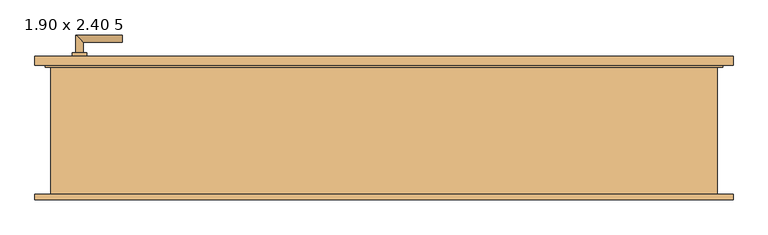
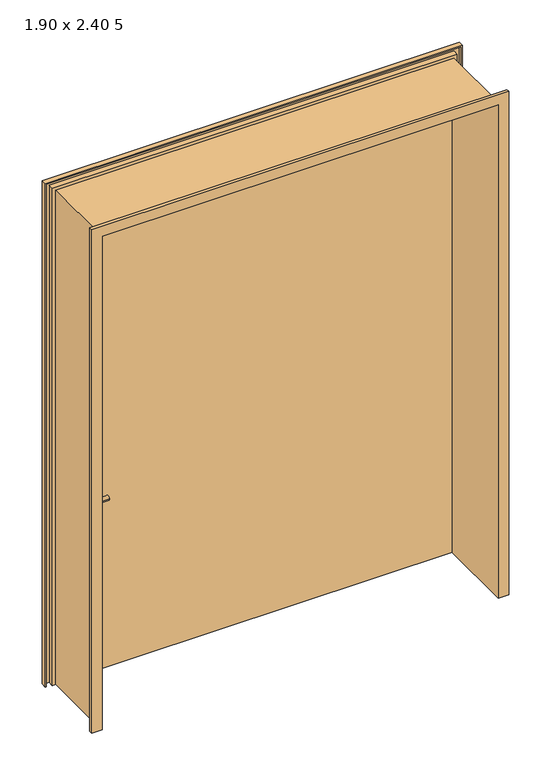
"""IFC4 building model written with IfcOpenShell, lengths in millimetres: door geometry, Drehflügel 1-flg - Stahlzarge : 1.90 x 2.40 5."""

from ifc_helpers import new_model, si_unit, point, frame, frame_2d, origin, place, context, project, spatial, polyline, circle_curve, ellipse_curve, trimmed, segment, composite_curve, outline, extrude, faceted_brep, source, transform, mapped, element, save
from ifc_brep_helpers import plane_surface, cylinder_surface, advanced_brep


def door_1_90_x_2_40_5_014a3839(model_context):
    return source(origin(), model_context, "Body", "SolidModel", [
        advanced_brep(
        [(-860.0, 169.4346141, 915.0), (-840.0, 169.4346141, 915.0), (-860.0, 99.4346141, 915.0), (-840.0, 119.4346141, 915.0), (-730.0, 99.4346141, 915.0), (-730.0, 119.4346141, 915.0)],
        [
            (0, 1, circle_curve(frame((-850.0, 169.4346141, 915.0), z_axis=(0.0, 1.0, 0.0), x_axis=(1.0, 0.0, 0.0)), 10.0)),
            (1, 0, circle_curve(frame((-850.0, 169.4346141, 915.0), z_axis=(0.0, 1.0, 0.0), x_axis=(1.0, 0.0, 0.0)), 10.0)),
            (0, 2),
            (2, 3, ellipse_curve(frame((-850.0, 109.4346141, 915.0), z_axis=(-0.7071067811865385, 0.7071067811865565, 0.0), x_axis=(0.7071067811865563, 0.7071067811865386, 0.0)), 14.1421356, 10.0)),
            (3, 1),
            (3, 2, ellipse_curve(frame((-850.0, 109.4346141, 915.0), z_axis=(-0.7071067811865385, 0.7071067811865565, 0.0), x_axis=(0.7071067811865563, 0.7071067811865386, 0.0)), 14.1421356, 10.0)),
            (4, 5, circle_curve(frame((-730.0, 109.4346141, 915.0), z_axis=(1.0, 0.0, 0.0), x_axis=(0.0, 1.0, 0.0)), 10.0)),
            (5, 4, circle_curve(frame((-730.0, 109.4346141, 915.0), z_axis=(1.0, 0.0, 0.0), x_axis=(0.0, 1.0, 0.0)), 10.0)),
            (2, 4),
            (5, 3),
        ],
        [
            plane_surface(frame((-850.0, 169.4346141, -372.7526403), z_axis=(0.0, 1.0, 0.0), x_axis=(0.0, 0.0, 1.0))),
            cylinder_surface(frame((-850.0, 169.4346141, 915.0), z_axis=(0.0, 1.0, 0.0), x_axis=(1.0, 0.0, 0.0)), 10.0),
            plane_surface(frame((-730.0, 109.4346141, -372.7526403), z_axis=(1.0, 0.0, 0.0), x_axis=(0.0, 0.0, 1.0))),
            cylinder_surface(frame((-850.0, 109.4346141, 915.0), z_axis=(-1.0, 0.0, 0.0), x_axis=(0.0, 1.0, 0.0)), 10.0),
        ],
        [
            (0, [[1, 2]]),
            (1, [[-1, 3, 4, 5]]),
            (1, [[-2, -5, 6, -3]]),
            (2, [[7, 8]]),
            (3, [[-4, 9, -8, 10]]),
            (3, [[-6, -10, -7, -9]]),
        ],
    ),
        advanced_brep(
        [(-840.0, 229.4346141, 915.0), (-860.0, 229.4346141, 915.0), (-840.0, 259.4346141, 915.0), (-860.0, 279.4346141, 915.0), (-730.0, 259.4346141, 915.0), (-730.0, 279.4346141, 915.0)],
        [
            (0, 1, circle_curve(frame((-850.0, 229.4346141, 915.0), z_axis=(0.0, -1.0, 0.0), x_axis=(-1.0, 0.0, 0.0)), 10.0)),
            (1, 0, circle_curve(frame((-850.0, 229.4346141, 915.0), z_axis=(0.0, -1.0, 0.0), x_axis=(-1.0, 0.0, 0.0)), 10.0)),
            (0, 2),
            (2, 3, ellipse_curve(frame((-850.0, 269.4346141, 915.0), z_axis=(-0.7071067811865475, -0.7071067811865475, 0.0), x_axis=(0.7071067811865474, -0.7071067811865476, 0.0)), 14.1421356, 10.0)),
            (3, 1),
            (3, 2, ellipse_curve(frame((-850.0, 269.4346141, 915.0), z_axis=(-0.7071067811865475, -0.7071067811865475, 0.0), x_axis=(0.7071067811865474, -0.7071067811865476, 0.0)), 14.1421356, 10.0)),
            (4, 5, circle_curve(frame((-730.0, 269.4346141, 915.0), z_axis=(1.0, 0.0, 0.0), x_axis=(0.0, 1.0, 0.0)), 10.0)),
            (5, 4, circle_curve(frame((-730.0, 269.4346141, 915.0), z_axis=(1.0, 0.0, 0.0), x_axis=(0.0, 1.0, 0.0)), 10.0)),
            (2, 4),
            (5, 3),
        ],
        [
            plane_surface(frame((-850.0, 229.4346141, -372.7526403), z_axis=(0.0, -1.0, 0.0), x_axis=(0.0, 0.0, 1.0))),
            cylinder_surface(frame((-850.0, 229.4346141, 915.0), z_axis=(0.0, -1.0, 0.0), x_axis=(-1.0, 0.0, 0.0)), 10.0),
            plane_surface(frame((-730.0, 269.4346141, -372.7526403), z_axis=(1.0, 0.0, 0.0), x_axis=(0.0, 0.0, 1.0))),
            cylinder_surface(frame((-850.0, 269.4346141, 915.0), z_axis=(-1.0, 0.0, 0.0), x_axis=(0.0, 1.0, 0.0)), 10.0),
        ],
        [
            (0, [[1, 2]]),
            (1, [[-1, 3, 4, 5]]),
            (1, [[-2, -5, 6, -3]]),
            (2, [[7, 8]]),
            (3, [[-4, 9, -8, 10]]),
            (3, [[-6, -10, -7, -9]]),
        ],
    ),
        extrude(outline(composite_curve([segment(trimmed(circle_curve(frame_2d((915.0, -850.0)), 20.0), [point((915.0, -870.0))], [point((915.0, -830.0))], False, "CARTESIAN"), True, "CONTINUOUS"), segment(trimmed(circle_curve(frame_2d((915.0, -850.0)), 20.0), [point((915.0, -830.0))], [point((915.0, -870.0))], False, "CARTESIAN"), True, "CONTINUOUS")], self_intersect=False)), frame((0.0, 159.4346141, 0.0), z_axis=(0.0, 1.0, 0.0), x_axis=(0.0, 0.0, 1.0)), (0.0, 0.0, 1.0), 10.0),
        extrude(outline(composite_curve([segment(trimmed(circle_curve(frame_2d((915.0, -850.0)), 20.0), [point((915.0, -870.0))], [point((915.0, -830.0))], False, "CARTESIAN"), True, "CONTINUOUS"), segment(trimmed(circle_curve(frame_2d((915.0, -850.0)), 20.0), [point((915.0, -830.0))], [point((915.0, -870.0))], False, "CARTESIAN"), True, "CONTINUOUS")], self_intersect=False)), frame((0.0, 219.4346141, 0.0), z_axis=(0.0, 1.0, 0.0), x_axis=(0.0, 0.0, 1.0)), (0.0, 0.0, 1.0), 10.0),
        extrude(outline(polyline([(940.0, 194.4346141), (-940.0, 194.4346141), (-940.0, 219.4346141), (940.0, 219.4346141), (940.0, 194.4346141)])), frame((0.0, 0.0, 15.0), z_axis=(0.0, 0.0, 1.0), x_axis=(1.0, 0.0, 0.0)), (0.0, 0.0, 1.0), 2450.0),
        faceted_brep([(974.4603207, -180.5653859, 15.0), (925.0, -180.5653859, 15.0), (925.0, 194.4346141, 15.0), (940.0, 194.4346141, 15.0), (940.0, 219.4346141, 15.0), (974.4603207, 219.4346141, 15.0), (974.4603207, 194.4346141, 15.0), (969.4603207, 194.4346141, 15.0), (969.4603207, 214.4346141, 15.0), (945.0, 214.4346141, 15.0), (945.0, 189.4346141, 15.0), (930.0, 189.4346141, 15.0), (930.0, -175.5653859, 15.0), (969.4603207, -175.5653859, 15.0), (969.4603207, -165.5653859, 15.0), (974.4603207, -165.5653859, 15.0), (974.4603207, -180.5653859, 2499.4603207), (-974.4603207, -180.5653859, 2499.4603207), (-974.4603207, -180.5653859, 15.0), (-925.0, -180.5653859, 15.0), (-925.0, -180.5653859, 2450.0), (925.0, -180.5653859, 2450.0), (925.0, 194.4346141, 2450.0), (-925.0, 194.4346141, 2450.0), (-925.0, 194.4346141, 15.0), (-940.0, 194.4346141, 15.0), (-940.0, 194.4346141, 2465.0), (940.0, 194.4346141, 2465.0), (940.0, 219.4346141, 2465.0), (-940.0, 219.4346141, 2465.0), (-940.0, 219.4346141, 15.0), (-974.4603207, 219.4346141, 15.0), (-974.4603207, 219.4346141, 2499.4603207), (974.4603207, 219.4346141, 2499.4603207), (974.4603207, 194.4346141, 2499.4603207), (-974.4603207, 194.4346141, 2499.4603207), (-974.4603207, 194.4346141, 15.0), (-969.4603207, 194.4346141, 15.0), (-969.4603207, 194.4346141, 2494.4603207), (969.4603207, 194.4346141, 2494.4603207), (969.4603207, 214.4346141, 2494.4603207), (-969.4603207, 214.4346141, 2494.4603207), (-969.4603207, 214.4346141, 15.0), (-945.0, 214.4346141, 15.0), (-945.0, 214.4346141, 2470.0), (945.0, 214.4346141, 2470.0), (945.0, 189.4346141, 2470.0), (-945.0, 189.4346141, 2470.0), (-945.0, 189.4346141, 15.0), (-930.0, 189.4346141, 15.0), (-930.0, 189.4346141, 2455.0), (930.0, 189.4346141, 2455.0), (930.0, -175.5653859, 2455.0), (-930.0, -175.5653859, 2455.0), (-930.0, -175.5653859, 15.0), (-969.4603207, -175.5653859, 15.0), (-969.4603207, -175.5653859, 2494.4603207), (969.4603207, -175.5653859, 2494.4603207), (969.4603207, -165.5653859, 2494.4603207), (-969.4603207, -165.5653859, 2494.4603207), (-969.4603207, -165.5653859, 15.0), (-974.4603207, -165.5653859, 15.0), (-974.4603207, -165.5653859, 2499.4603207), (974.4603207, -165.5653859, 2499.4603207)], [[[0, 1, 2, 3, 4, 5, 6, 7, 8, 9, 10, 11, 12, 13, 14, 15]], [[1, 0, 16, 17, 18, 19, 20, 21]], [[2, 1, 21, 22]], [[3, 2, 22, 23, 24, 25, 26, 27]], [[4, 3, 27, 28]], [[5, 4, 28, 29, 30, 31, 32, 33]], [[6, 5, 33, 34]], [[7, 6, 34, 35, 36, 37, 38, 39]], [[8, 7, 39, 40]], [[9, 8, 40, 41, 42, 43, 44, 45]], [[10, 9, 45, 46]], [[11, 10, 46, 47, 48, 49, 50, 51]], [[12, 11, 51, 52]], [[13, 12, 52, 53, 54, 55, 56, 57]], [[14, 13, 57, 58]], [[15, 14, 58, 59, 60, 61, 62, 63]], [[0, 15, 63, 16]], [[17, 62, 61, 18]], [[18, 61, 60, 55, 54, 49, 48, 43, 42, 37, 36, 31, 30, 25, 24, 19]], [[23, 20, 19, 24]], [[29, 26, 25, 30]], [[35, 32, 31, 36]], [[41, 38, 37, 42]], [[47, 44, 43, 48]], [[53, 50, 49, 54]], [[59, 56, 55, 60]], [[22, 21, 20, 23]], [[28, 27, 26, 29]], [[34, 33, 32, 35]], [[40, 39, 38, 41]], [[46, 45, 44, 47]], [[52, 51, 50, 53]], [[58, 57, 56, 59]], [[16, 63, 62, 17]]]),
    ])


if __name__ == "__main__":
    model = new_model("IFC4")
    model_context = context("Model", 3, world=origin())
    ifc_project = project(units=[si_unit("LENGTHUNIT", "METRE", prefix="MILLI")], contexts=[model_context])
    site = spatial("IfcSite", under=ifc_project)
    building = spatial("IfcBuilding", under=site)
    placement = place(None, origin())
    door_1_90_x_2_40_5_shape = door_1_90_x_2_40_5_014a3839(model_context)
    element("IfcDoor", 1, ObjectType="Drehflügel 1-flg - Stahlzarge : 1.90 x 2.40 5", at=placement, inside=building, context=model_context, shape_type="MappedRepresentation", body=[
        mapped(door_1_90_x_2_40_5_shape, transform((0.0, 0.0, 0.0), x_axis=(1.0, 0.0, 0.0), y_axis=(0.0, 1.0, 0.0), z_axis=(0.0, 0.0, 1.0))),
    ])
    save(model, "model.ifc")

# Revit data of these elements
# Type "Drehflügel 1-flg - Stahlzarge : 1.90 x 2.40 5"
#   Type Mark = "27"
#   Operation = "SingleSwingRight"
#   Keynote = "16.03"
#   Analytic Construction = "Metall"
#   Thermal Resistance (R) = 0.270117 (m²·K)/W
#   Heat Transfer Coefficient (U) = 3.7021 W/(m²·K)
#   Rough Width = 1.900 m
#   Rough Height [instance default] = 2.560 m
#   Höhe Türgriff [instance default] = 0.900 m
#   Height = 2.460 m
#   Fußbodenaufbau [instance default] = 0.100 m
#   Width = 1.900 m
#   Sichtbarkeit Sturzlinien [instance default] = yes
#   Türgriff auswählen [instance default] = element 221079
#   Türgriff [instance default] = none
#   Türflügel [instance default] = none
#   Rahmen/Pfosten [instance default] = Metall - Lackiert - Grau
#   Visual Light Transmittance = 0
#   Solar Heat Gain Coefficient = 0
#   Function = (empty or 0)
#   Wall Closure = (empty or 0)
# Element 1 (IfcDoor, "Drehflügel 1-flg - Stahlzarge : 1.90 x 2.40 5")
#   Rough Height = 2.475 m
#   Fußbodenaufbau = 0.015 m
#   Materials on its faces: "Metall - Lackiert - Grau", "Metall - Chrom", "Holz - Birke"
# Materials
#   "Metall - Lackiert - Grau": class "Farbe 1", colour RGB 98 98 98, transparency 0, Cost = 0
#   "Metall - Chrom": class "Metall", colour RGB 247 247 247, transparency 0, Cost = 0
#   "Holz - Birke": class "Holz", colour RGB 213 164 103, transparency 0, Cost = 0
